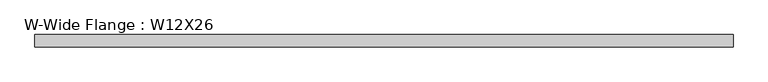
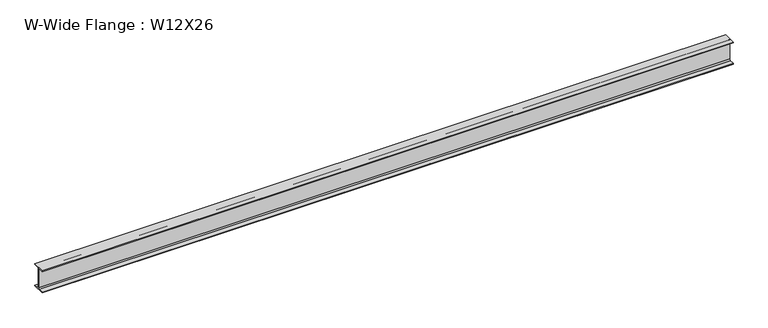
"""IFC4 building model written with IfcOpenShell, lengths in millimetres: beam geometry, W-Wide Flange : W12X26."""

from ifc_helpers import new_model, si_unit, point, frame, frame_2d, origin, place, context, project, spatial, polyline, circle_curve, trimmed, segment, composite_curve, outline, extrude, source, transform, mapped, element, save


def w_wide_flange_w12x26_d1c4accc(model_context):
    return source(origin(), model_context, "Body", "SweptSolid", [
        extrude(outline(composite_curve([segment(polyline([(82.423, -145.288), (82.423, -154.94), (-82.423, -154.94), (-82.423, -145.288), (-20.2565, -145.288)]), True, "CONTINUOUS"), segment(trimmed(circle_curve(frame_2d((-20.2565, -127.9525)), 17.3355), [point((-20.2565, -145.288))], [point((-2.921, -127.9525))], True, "CARTESIAN"), True, "CONTINUOUS"), segment(polyline([(-2.921, -127.9525), (-2.921, 127.9525)]), True, "CONTINUOUS"), segment(trimmed(circle_curve(frame_2d((-20.2565, 127.9525)), 17.3355), [point((-2.921, 127.9525))], [point((-20.2565, 145.288))], True, "CARTESIAN"), True, "CONTINUOUS"), segment(polyline([(-20.2565, 145.288), (-82.423, 145.288), (-82.423, 154.94), (82.423, 154.94), (82.423, 145.288), (20.2565, 145.288)]), True, "CONTINUOUS"), segment(trimmed(circle_curve(frame_2d((20.2565, 127.9525)), 17.3355), [point((20.2565, 145.288))], [point((2.921, 127.9525))], True, "CARTESIAN"), True, "CONTINUOUS"), segment(polyline([(2.921, 127.9525), (2.921, -127.9525)]), True, "CONTINUOUS"), segment(trimmed(circle_curve(frame_2d((20.2565, -127.9525)), 17.3355), [point((2.921, -127.9525))], [point((20.2565, -145.288))], True, "CARTESIAN"), True, "CONTINUOUS"), segment(polyline([(20.2565, -145.288), (82.423, -145.288)]), True, "CONTINUOUS")], self_intersect=False)), frame((-4587.95401, 0.0, 0.0), z_axis=(1.0, 0.0, 0.0), x_axis=(0.0, 1.0, 0.0)), (0.0, 0.0, 1.0), 9207.5),
    ])


if __name__ == "__main__":
    model = new_model("IFC4")
    model_context = context("Model", 3, world=origin())
    ifc_project = project(units=[si_unit("LENGTHUNIT", "METRE", prefix="MILLI")], contexts=[model_context])
    site = spatial("IfcSite", under=ifc_project)
    building = spatial("IfcBuilding", under=site)
    placement = place(None, origin())
    w_wide_flange_w12x26_shape = w_wide_flange_w12x26_d1c4accc(model_context)
    element("IfcBeam", 1, ObjectType="W-Wide Flange : W12X26", at=placement, inside=building, context=model_context, shape_type="MappedRepresentation", body=[
        mapped(w_wide_flange_w12x26_shape, transform((0.0, 0.0, 0.0), x_axis=(1.0, 0.0, 0.0), y_axis=(0.0, 1.0, 0.0), z_axis=(0.0, 0.0, 1.0))),
    ])
    save(model, "model.ifc")

# Revit data of these elements
# Type "W-Wide Flange : W12X26"
#   Assembly Code = "B10"
#   W = 26
#   Length [instance default] = 5' - 0"
#   bf = 0' - 6.49"
#   d = 1' - 0.2"
#   k = 0' - 1 1/16"
#   k2 = 0' - 0.6825"
#   tf = 0' - 0.38"
#   tw = 0' - 0.23"
#   A = 0.053125 SF
#   Structural Material [instance default] = Steel ASTM A992
# Element 1 (IfcBeam, "W-Wide Flange : W12X26")
#   Materials on its faces: "Steel ASTM A992"
# Materials
#   "Steel ASTM A992": class "Metal", colour RGB 199 199 199, transparency 0, Description = "Structural steel 50ksi", Cost = 0
